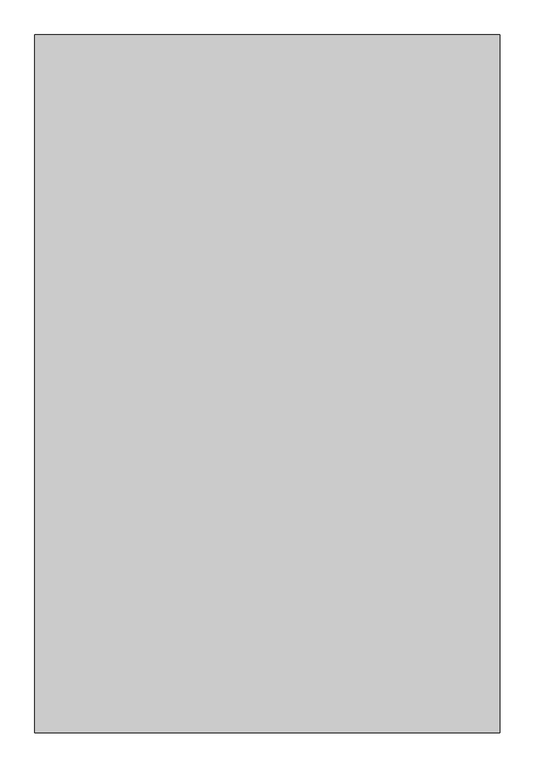
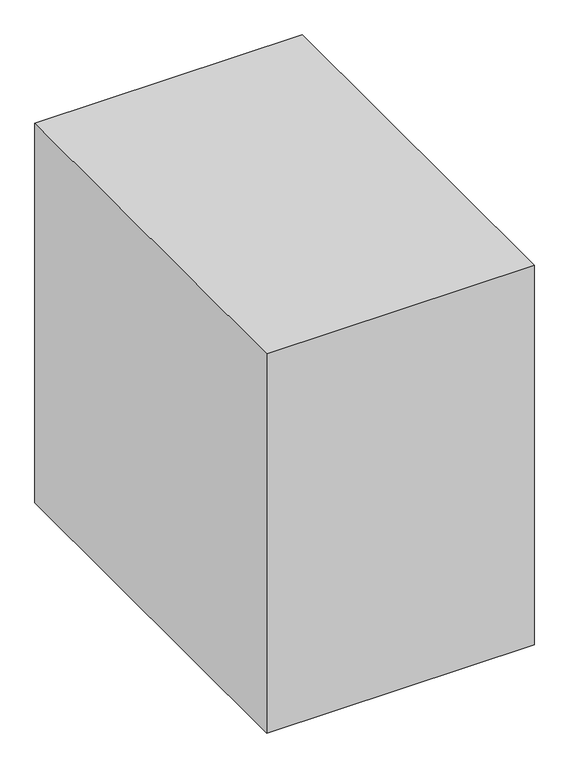
"""IFC4 building model written with IfcOpenShell, lengths in millimetres: proxy geometry, Space Planning Box_hec : Space Planning Box_hec."""

import ifcopenshell
import ifcopenshell.guid

model = None  # the IFC model being written
_history = None  # IfcOwnerHistory: only IFC2X3 demands one
_inside = {}  # id of a spatial element -> (the spatial element, [elements in it])
_under = {}  # id of a project, library or spatial element -> (it, [spatial elements below it])
_declared = {}  # id of a project -> (the project, [libraries it declares])
_typed = {}  # id of a type object -> (the type object, [elements of that type])
_made_of = {}  # id of a material, layer set ... -> (it, [elements and type objects made of it])


def new_model(schema):
    """Start an empty IFC model of exactly this schema.

    Asked for "IFC4X3", IfcOpenShell would pick the latest addendum, in which some entities
    have other attributes; the version numbers below select the first issue.
    IFC2X3 requires an IfcOwnerHistory on every rooted entity: one is made here for all.
    """
    global model, _history
    if schema == "IFC4X3":
        model = ifcopenshell.file(schema_version=(4, 3, 0, 0))
    else:
        model = ifcopenshell.file(schema=schema)
    _inside.clear()
    _under.clear()
    _declared.clear()
    _typed.clear()
    _made_of.clear()
    _history = None
    if model.schema == "IFC2X3":
        org = make("IfcOrganization", Name="unknown")
        user = make(
            "IfcPersonAndOrganization",
            ThePerson=make("IfcPerson", FamilyName="unknown"),
            TheOrganization=org,
        )
        app = make(
            "IfcApplication",
            ApplicationDeveloper=org,
            Version="unknown",
            ApplicationFullName="unknown",
            ApplicationIdentifier="unknown",
        )
        _history = make(
            "IfcOwnerHistory",
            OwningUser=user,
            OwningApplication=app,
            ChangeAction="ADDED",
            CreationDate=0,
        )
    return model


def make(cls, **values):
    """One entity of the class cls with the attributes given. An attribute that is None is left unset."""
    return model.create_entity(
        cls, **{name: value for name, value in values.items() if value is not None}
    )


def rooted(cls, **values):
    """An entity with a GlobalId (a new one), such as an element, a storey or a relation."""
    return make(cls, GlobalId=ifcopenshell.guid.new(), OwnerHistory=_history, **values)


def si_unit(unit_type, name, prefix=None):
    """IfcSIUnit, for example si_unit("LENGTHUNIT", "METRE", prefix="MILLI")."""
    return make("IfcSIUnit", UnitType=unit_type, Prefix=prefix, Name=name)


def assignment(units):
    """IfcUnitAssignment: the units of a project."""
    return None if units is None else make("IfcUnitAssignment", Units=units)


def point(xyz):
    """IfcCartesianPoint."""
    return None if xyz is None else make("IfcCartesianPoint", Coordinates=xyz)


def direction(xyz):
    """IfcDirection."""
    return None if xyz is None else make("IfcDirection", DirectionRatios=xyz)


def frame(location, z_axis=None, x_axis=None):
    """IfcAxis2Placement3D, a coordinate frame: its origin and axes. An axis left out is left unset."""
    return make(
        "IfcAxis2Placement3D",
        Location=point(location),
        Axis=direction(z_axis),
        RefDirection=direction(x_axis),
    )


def origin():
    """The frame at (0, 0, 0) with its axes left unset."""
    return frame((0.0, 0.0, 0.0))


def origin_with_axes():
    """The frame at (0, 0, 0) with the z axis (0, 0, 1) and the x axis (1, 0, 0) written out."""
    return frame((0.0, 0.0, 0.0), z_axis=(0.0, 0.0, 1.0), x_axis=(1.0, 0.0, 0.0))


def place(relative_to, where):
    """IfcLocalPlacement: puts the frame where relative to a parent placement (None: the world)."""
    return make(
        "IfcLocalPlacement", PlacementRelTo=relative_to, RelativePlacement=where
    )


def context(
    kind, dimensions, precision=None, world=None, true_north=None, identifier=None
):
    """IfcGeometricRepresentationContext, for example the 3D "Model" context."""
    return make(
        "IfcGeometricRepresentationContext",
        ContextIdentifier=identifier,
        ContextType=kind,
        CoordinateSpaceDimension=dimensions,
        Precision=precision,
        WorldCoordinateSystem=world,
        TrueNorth=true_north,
    )


def project(units=None, contexts=None):
    """IfcProject with its units and contexts."""
    return rooted(
        "IfcProject",
        Name="project",
        RepresentationContexts=contexts,
        UnitsInContext=assignment(units),
    )


def spatial(cls, under=None, at=None, **own):
    """A site, building, storey or space (cls), placed at a placement, below another one or the project."""
    s = rooted(cls, ObjectPlacement=at, **own)
    if under is not None:
        _under.setdefault(under.id(), (under, []))[1].append(s)
    return s


def polyline(points):
    """IfcPolyline through the points."""
    return make("IfcPolyline", Points=[point(p) for p in points])


def outline(outer, holes=None, kind="AREA"):
    """IfcArbitraryClosedProfileDef: a profile drawn as a closed curve; with holes, ...WithVoids."""
    if holes is None:
        return make("IfcArbitraryClosedProfileDef", ProfileType=kind, OuterCurve=outer)
    return make(
        "IfcArbitraryProfileDefWithVoids",
        ProfileType=kind,
        OuterCurve=outer,
        InnerCurves=holes,
    )


def extrude(swept, where, along, depth):
    """IfcExtrudedAreaSolid: the profile swept, set in the frame where, extruded along a direction by depth."""
    return make(
        "IfcExtrudedAreaSolid",
        SweptArea=swept,
        Position=where,
        ExtrudedDirection=direction(along),
        Depth=depth,
    )


def shape(context_of_items, identifier, shape_type, items):
    """IfcShapeRepresentation: the items that make up one representation, for example the "Body"."""
    return make(
        "IfcShapeRepresentation",
        ContextOfItems=context_of_items,
        RepresentationIdentifier=identifier,
        RepresentationType=shape_type,
        Items=items,
    )


def source(mapping_origin, context_of_items, identifier, shape_type, items):
    """IfcRepresentationMap: a shape defined once, which mapped items show again and again."""
    return make(
        "IfcRepresentationMap",
        MappingOrigin=mapping_origin,
        MappedRepresentation=shape(context_of_items, identifier, shape_type, items),
    )


def transform(
    local_origin,
    x_axis=None,
    y_axis=None,
    z_axis=None,
    scale=None,
    scale2=None,
    scale3=None,
    uniform=True,
):
    """IfcCartesianTransformationOperator3D, or its non-uniform kind. x_axis, y_axis, z_axis: its Axis1, 2, 3."""
    if uniform:
        return make(
            "IfcCartesianTransformationOperator3D",
            Axis1=direction(x_axis),
            Axis2=direction(y_axis),
            LocalOrigin=point(local_origin),
            Scale=scale,
            Axis3=direction(z_axis),
        )
    return make(
        "IfcCartesianTransformationOperator3DnonUniform",
        Axis1=direction(x_axis),
        Axis2=direction(y_axis),
        LocalOrigin=point(local_origin),
        Scale=scale,
        Axis3=direction(z_axis),
        Scale2=scale2,
        Scale3=scale3,
    )


def mapped(mapping_source, mapping_target):
    """IfcMappedItem: shows the shape of a source again, moved by a transform."""
    return make(
        "IfcMappedItem", MappingSource=mapping_source, MappingTarget=mapping_target
    )


def made_of(thing, what):
    """Note that an element or type object is made of a material, layer set ...; save() writes the relation."""
    if what is not None:
        _made_of.setdefault(what.id(), (what, []))[1].append(thing)
    return thing


def element(
    cls,
    number,
    at=None,
    inside=None,
    cuts=None,
    type_object=None,
    material=None,
    context=None,
    identifier="Body",
    shape_type=None,
    held_by="IfcProductDefinitionShape",
    body=None,
    shapes=None,
    **own,
):
    """One element of the class cls, such as IfcWall. Its Tag is "e" and its number.

    at: its placement. inside: the storey or other place that contains it. cuts: it is an
    opening in that element (IfcRelVoidsElement). A single representation is given by context,
    identifier, shape_type and body (its items); several are given by shapes. held_by: the class
    of the entity that holds the representations. save() writes the other relations.
    """
    e = rooted(cls, Tag="e%d" % number, ObjectPlacement=at, **own)
    if body is not None:
        shapes = [shape(context, identifier, shape_type, body)]
    if shapes is not None:
        e.Representation = make(held_by, Representations=shapes)
    if inside is not None:
        _inside.setdefault(inside.id(), (inside, []))[1].append(e)
    if cuts is not None:
        rooted(
            "IfcRelVoidsElement", RelatingBuildingElement=cuts, RelatedOpeningElement=e
        )
    if type_object is not None:
        _typed.setdefault(type_object.id(), (type_object, []))[1].append(e)
    return made_of(e, material)


def aggregate(whole, parts):
    """IfcRelAggregates: a whole, such as a stair, and the parts it consists of."""
    return rooted("IfcRelAggregates", RelatingObject=whole, RelatedObjects=parts)


def save(model, path):
    """Write the relations noted so far, then the file.

    IfcRelAggregates (storeys below a building ...), IfcRelContainedInSpatialStructure (elements
    in a storey), IfcRelDefinesByType, IfcRelAssociatesMaterial and IfcRelDeclares: one each for
    every whole, place, type object, material and project.
    """
    for whole, parts in _under.values():
        aggregate(whole, parts)
    for where, things in _inside.values():
        rooted(
            "IfcRelContainedInSpatialStructure",
            RelatedElements=things,
            RelatingStructure=where,
        )
    for kind, things in _typed.values():
        rooted("IfcRelDefinesByType", RelatedObjects=things, RelatingType=kind)
    for what, things in _made_of.values():
        rooted("IfcRelAssociatesMaterial", RelatedObjects=things, RelatingMaterial=what)
    for by, libraries in _declared.values():
        rooted("IfcRelDeclares", RelatingContext=by, RelatedDefinitions=libraries)
    model.write(path)


def generic_models_98b71764(model_context):
    return source(origin(), model_context, "Body", "SweptSolid", [
        extrude(outline(polyline([(2000.0, 3000.0), (2000.0, -3000.0), (-2000.0, -3000.0), (-2000.0, 3000.0), (2000.0, 3000.0)])), origin_with_axes(), (0.0, 0.0, 1.0), 6000.0),
    ])


if __name__ == "__main__":
    model = new_model("IFC4")
    model_context = context("Model", 3, world=origin())
    ifc_project = project(units=[si_unit("LENGTHUNIT", "METRE", prefix="MILLI")], contexts=[model_context])
    site = spatial("IfcSite", under=ifc_project)
    building = spatial("IfcBuilding", under=site)
    placement = place(None, origin())
    generic_models_shape = generic_models_98b71764(model_context)
    element("IfcBuildingElementProxy", 1, Name="Space Planning Box_hec : Space Planning Box_hec", ObjectType="Space Planning Box_hec : Space Planning Box_hec", at=placement, inside=building, context=model_context, shape_type="MappedRepresentation", body=[
        mapped(generic_models_shape, transform((0.0, 0.0, 0.0), x_axis=(1.0, 0.0, 0.0), y_axis=(0.0, 1.0, 0.0), z_axis=(0.0, 0.0, 1.0))),
    ])
    save(model, "model.ifc")

# Revit data of these elements
# Type "Space Planning Box_hec : Space Planning Box_hec"
#   Type Comments = "..."
#   Room Name [instance default] = "?"
#   Interior Finish [instance default] = ""
#   Exterior Finish [instance default] = ""
#   Department [instance default] = ""
#   Assembly Code = "..."
#   Width [instance default] = 1524 mm
#   Program Area [instance default] = 0.00 m²
#   Length [instance default] = 1524 mm
#   Height [instance default] = 1524 mm
#   Area [instance default] = 2.32258 m²
#   Fill Color [instance default] = Cyan
#   Default Elevation = 0
# Element 1 (IfcBuildingElementProxy, "Space Planning Box_hec : Space Planning Box_hec")
#   Room Name = "Shift Office Room"
#   Interior Finish = "IF2-1"
#   Exterior Finish = "EF1"
#   Department = "AR"
#   Width = 4000 mm
#   Program Area = 43.20 m²
#   Length = 6000 mm
#   Height = 6000 mm
#   Area = 24.00 m²
#   Fill Color = Lavender
#   Materials on its faces: "Lavender"
# Materials
#   "Cyan": class "Generic", colour RGB 0 255 255, transparency 0.2, Cost = 0
#   "Lavender": class "Generic", colour RGB 186 85 211, transparency 0.2, Cost = 0
